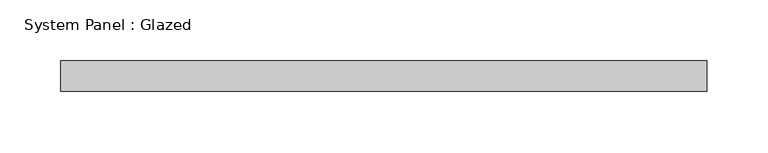
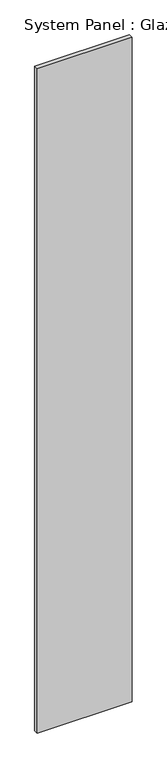
"""IFC4 building model written with IfcOpenShell, lengths in millimetres: plate geometry, System Panel : Glazed."""

from ifc_helpers import new_model, si_unit, origin, origin_with_axes, place, context, project, spatial, polyline, outline, extrude, source, transform, mapped, element, save


def system_panel_glazed_f8c549d9(model_context):
    return source(origin(), model_context, "Body", "SweptSolid", [
        extrude(outline(polyline([(266.25, 24.5), (-266.25, 24.5), (-266.25, 49.5), (266.25, 49.5), (266.25, 24.5)])), origin_with_axes(), (0.0, 0.0, 1.0), 3950.0),
    ])


if __name__ == "__main__":
    model = new_model("IFC4")
    model_context = context("Model", 3, world=origin())
    ifc_project = project(units=[si_unit("LENGTHUNIT", "METRE", prefix="MILLI")], contexts=[model_context])
    site = spatial("IfcSite", under=ifc_project)
    building = spatial("IfcBuilding", under=site)
    placement = place(None, origin())
    system_panel_glazed_shape = system_panel_glazed_f8c549d9(model_context)
    element("IfcPlate", 1, ObjectType="System Panel : Glazed", at=placement, inside=building, context=model_context, shape_type="MappedRepresentation", body=[
        mapped(system_panel_glazed_shape, transform((0.0, 0.0, 0.0), x_axis=(1.0, 0.0, 0.0), y_axis=(0.0, 1.0, 0.0), z_axis=(0.0, 0.0, 1.0))),
    ])
    save(model, "model.ifc")

# Revit data of these elements
# Type "System Panel : Glazed"
#   Keynote = "H11"
#   Construction Type Id = "GSP4R"
#   Analytic Construction = "1/8 in Pilkington single glazing"
#   Visual Light Transmittance = 0.9
#   Solar Heat Gain Coefficient = 0.86
#   Heat Transfer Coefficient (U) = 6.7069 W/(m²·K)
#   Define Thermal Properties by = 1
# Element 1 (IfcPlate, "System Panel : Glazed")
#   Materials on its faces: "Glass"
# Materials
#   "Glass": class "Glass", colour RGB 0 128 192, transparency 0.9, Description = "Soda Lime Glass", Cost = 0
